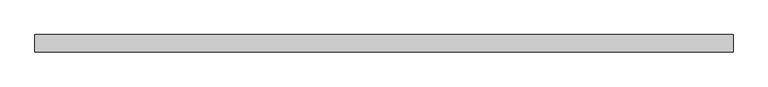
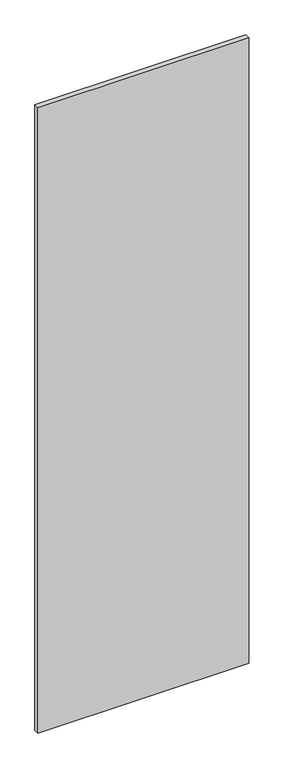
"""IFC4 building model written with IfcOpenShell, lengths in millimetres: plate geometry, 系统嵌板 : 玻璃."""

from ifc_helpers import new_model, si_unit, origin, origin_with_axes, place, context, project, spatial, polyline, outline, extrude, source, transform, mapped, element, save


def plate_eba9dd67(model_context):
    return source(origin(), model_context, "Body", "SweptSolid", [
        extrude(outline(polyline([(510.0, -12.5), (-510.0, -12.5), (-510.0, 12.5), (510.0, 12.5), (510.0, -12.5)])), origin_with_axes(), (0.0, 0.0, 1.0), 3200.0),
    ])


if __name__ == "__main__":
    model = new_model("IFC4")
    model_context = context("Model", 3, world=origin())
    ifc_project = project(units=[si_unit("LENGTHUNIT", "METRE", prefix="MILLI")], contexts=[model_context])
    site = spatial("IfcSite", under=ifc_project)
    building = spatial("IfcBuilding", under=site)
    placement = place(None, origin())
    plate_shape = plate_eba9dd67(model_context)
    element("IfcPlate", 1, ObjectType="系统嵌板 : 玻璃", at=placement, inside=building, context=model_context, shape_type="MappedRepresentation", body=[
        mapped(plate_shape, transform((0.0, 0.0, 0.0), x_axis=(1.0, 0.0, 0.0), y_axis=(0.0, 1.0, 0.0), z_axis=(0.0, 0.0, 1.0))),
    ])
    save(model, "model.ifc")

# Revit data of these elements
# Type "系统嵌板 : 玻璃"
#   Construction Type Id = "GSP4R"
#   Analytic Construction = "1/8 英寸 Pilkington 单层玻璃"
#   Visual Light Transmittance = 0.9
#   Solar Heat Gain Coefficient = 0.86
#   Heat Transfer Coefficient (U) = 6.7069 W/(m²·K)
# Element 1 (IfcPlate, "系统嵌板 : 玻璃")
#   Materials on its faces: "玻璃"
# Materials
#   "玻璃": class "玻璃", colour RGB 0 128 192, transparency 0.9, Description = "钠钙玻璃", Cost = 0
